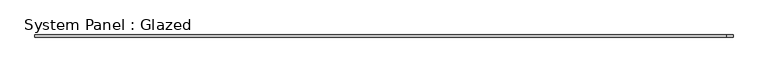
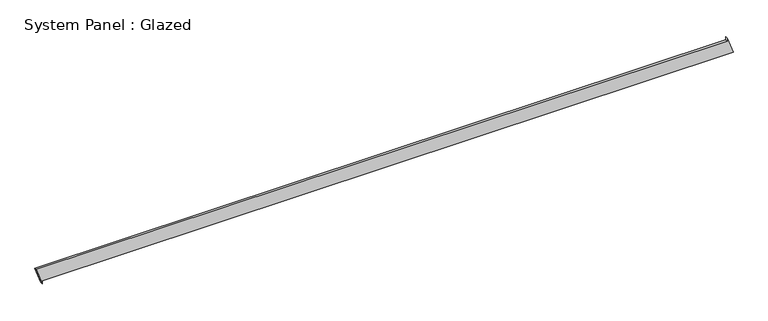
"""IFC4 building model written with IfcOpenShell, lengths in millimetres: plate geometry, System Panel : Glazed."""

from ifc_helpers import new_model, si_unit, frame, origin, place, context, project, spatial, polyline, outline, extrude, source, transform, mapped, element, save


def system_panel_glazed_fe5ea76c(model_context):
    return source(origin(), model_context, "Body", "SweptSolid", [
        extrude(outline(polyline([(0.0, -3956.7629895), (35.3553391, -3956.7629895), (35.3553391, 4027.1398136), (235.0472205, 3956.767991), (199.6918814, 3956.7680004), (199.6897639, -4027.1398136), (0.0, -3956.7629895)])), frame((0.0, -49.5, 0.0), z_axis=(0.0, 1.0, 0.0), x_axis=(0.0, 0.0, 1.0)), (0.0, 0.0, 1.0), 25.0),
    ])


if __name__ == "__main__":
    model = new_model("IFC4")
    model_context = context("Model", 3, world=origin())
    ifc_project = project(units=[si_unit("LENGTHUNIT", "METRE", prefix="MILLI")], contexts=[model_context])
    site = spatial("IfcSite", under=ifc_project)
    building = spatial("IfcBuilding", under=site)
    placement = place(None, origin())
    system_panel_glazed_shape = system_panel_glazed_fe5ea76c(model_context)
    element("IfcPlate", 1, ObjectType="System Panel : Glazed", at=placement, inside=building, context=model_context, shape_type="MappedRepresentation", body=[
        mapped(system_panel_glazed_shape, transform((0.0, 0.0, 0.0), x_axis=(1.0, 0.0, 0.0), y_axis=(0.0, 1.0, 0.0), z_axis=(0.0, 0.0, 1.0))),
    ])
    save(model, "model.ifc")

# Revit data of these elements
# Element 1 (IfcPlate, "System Panel : Glazed")
#   Materials on its faces: "Glass"
# Materials
#   "Glass": class "Glass", colour RGB 218 227 224, transparency 0.85, Description = "Soda Lime Glass", Cost = 0
